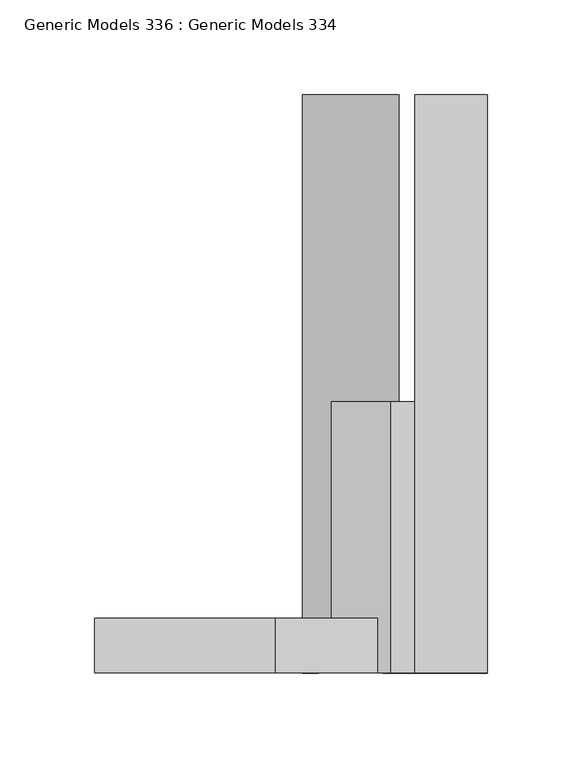
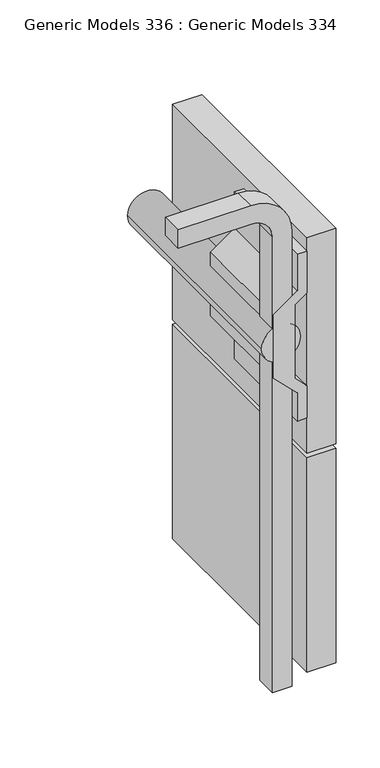
"""IFC4 building model written with IfcOpenShell, lengths in millimetres: proxy geometry, Generic Models 336 : Generic Models 334."""

from ifc_helpers import new_model, si_unit, point, frame, frame_2d, origin, place, context, project, spatial, polyline, circle_curve, trimmed, segment, composite_curve, outline, extrude, source, transform, mapped, element, save


def generic_models_336_generic_models_334_61ed0e0d(model_context):
    return source(origin(), model_context, "Body", "SweptSolid", [
        extrude(outline(polyline([(124298.119347, 8247.7371996), (124355.269347, 8247.7371996), (124355.269347, 8235.0371996), (124304.7305486, 8235.0371996), (124282.8772864, 8203.8275067), (124194.8055726, 8203.8275067), (124163.5958797, 8235.0371996), (124124.4063919, 8235.0371996), (124124.4063919, 8247.7371996), (124168.8563919, 8247.7371996), (124184.8192908, 8231.7743007), (124286.9420049, 8231.7743007), (124298.119347, 8247.7371996)])), frame((0.0, -4109.6428838, 0.0), z_axis=(0.0, 1.0, 0.0), x_axis=(0.0, 0.0, 1.0)), (0.0, 0.0, 1.0), 143.0193921),
        extrude(outline(composite_curve([segment(trimmed(circle_curve(frame_2d((124240.6161869, 8213.7932071)), 25.4), [point((124240.6161869, 8239.1932071))], [point((124240.6161869, 8188.3932071))], False, "CARTESIAN"), True, "CONTINUOUS"), segment(trimmed(circle_curve(frame_2d((124240.6161869, 8213.7932071)), 25.4), [point((124240.6161869, 8188.3932071))], [point((124240.6161869, 8239.1932071))], False, "CARTESIAN"), True, "CONTINUOUS")], self_intersect=False)), frame((0.0, -4109.6428838, 0.0), z_axis=(0.0, 1.0, 0.0), x_axis=(0.0, 0.0, 1.0)), (0.0, 0.0, 1.0), 304.8),
        extrude(outline(composite_curve([segment(trimmed(circle_curve(frame_2d((124390.2878103, 8174.0354038)), 53.8815367), [point((124390.2878103, 8227.9169406))], [point((124444.169347, 8174.0354038))], False, "CARTESIAN"), True, "CONTINUOUS"), segment(polyline([(124444.169347, 8174.0354038), (124444.169347, 8078.7854038), (124418.769347, 8078.7854038), (124418.769347, 8174.0354038)]), True, "CONTINUOUS"), segment(trimmed(circle_curve(frame_2d((124390.2878103, 8174.0354038)), 28.4815367), [point((124418.769347, 8174.0354038))], [point((124390.2878103, 8202.5169406))], True, "CARTESIAN"), True, "CONTINUOUS"), segment(polyline([(124390.2878103, 8202.5169406), (123759.5598344, 8202.5169406), (123759.5598344, 8227.9169406), (124390.2878103, 8227.9169406)]), True, "CONTINUOUS")], self_intersect=False)), frame((0.0, -4109.6428838, 0.0), z_axis=(0.0, 1.0, 0.0), x_axis=(0.0, 0.0, 1.0)), (0.0, 0.0, 1.0), 28.9445755),
        extrude(outline(polyline([(8247.7371996, -3804.8428838), (8285.8371996, -3804.8428838), (8285.8371996, -4109.6428838), (8247.7371996, -4109.6428838), (8247.7371996, -3804.8428838)])), frame((0.0, 0.0, 123771.8971121), z_axis=(0.0, 0.0, 1.0), x_axis=(1.0, 0.0, 0.0)), (0.0, 0.0, 1.0), 297.3238879),
        extrude(outline(polyline([(8247.7371996, -3804.8428838), (8285.8371996, -3804.8428838), (8285.8371996, -4109.6428838), (8247.7371996, -4109.6428838), (8247.7371996, -3804.8428838)])), frame((0.0, 0.0, 124075.571), z_axis=(0.0, 0.0, 1.0), x_axis=(1.0, 0.0, 0.0)), (0.0, 0.0, 1.0), 298.45),
    ])


if __name__ == "__main__":
    model = new_model("IFC4")
    model_context = context("Model", 3, world=origin())
    ifc_project = project(units=[si_unit("LENGTHUNIT", "METRE", prefix="MILLI")], contexts=[model_context])
    site = spatial("IfcSite", under=ifc_project)
    building = spatial("IfcBuilding", under=site)
    placement = place(None, origin())
    generic_models_336_generic_models_334_shape = generic_models_336_generic_models_334_61ed0e0d(model_context)
    element("IfcBuildingElementProxy", 1, Name="Generic Models 336 : Generic Models 334", ObjectType="Generic Models 336 : Generic Models 334", at=placement, inside=building, context=model_context, shape_type="MappedRepresentation", body=[
        mapped(generic_models_336_generic_models_334_shape, transform((0.0, 0.0, 0.0), x_axis=(1.0, 0.0, 0.0), y_axis=(0.0, 1.0, 0.0), z_axis=(0.0, 0.0, 1.0))),
    ])
    save(model, "model.ifc")

# Revit data of these elements
# Element 1 (IfcBuildingElementProxy, "Generic Models 336 : Generic Models 334")
#   Materials on its faces: "_GARAGE DOOR TRACK", "_SECTIONAL WOODEN GARAGE DOOR PER SCHEDULE"
# Materials
#   "_GARAGE DOOR TRACK": class "Metal", colour RGB 199 199 199, transparency 0, Description = "Structural steel 50ksi", Cost = 0
#   "_SECTIONAL WOODEN GARAGE DOOR PER SCHEDULE": class "Generic", colour RGB 177 130 114, transparency 0, Cost = 0
